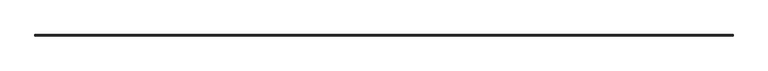
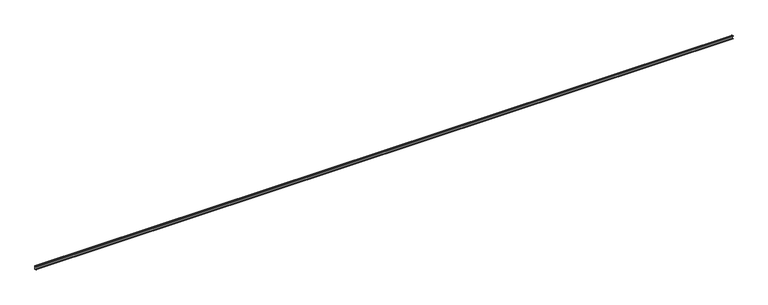
"""IFC4 building model written with IfcOpenShell, lengths in millimetres: beam geometry, 0912_Steel Framing_LC_KDS3530 : H_SB_AR_B03_LC-200x75x25x3.2."""

from ifc_helpers import new_model, si_unit, point, frame, frame_2d, origin, place, context, project, spatial, polyline, circle_curve, trimmed, segment, composite_curve, outline, extrude, source, transform, mapped, element, save


def beam_ae6eba6b(model_context):
    return source(origin(), model_context, "Body", "SweptSolid", [
        extrude(outline(composite_curve([segment(polyline([(18.6, 87.5), (18.6, -87.5)]), True, "CONTINUOUS"), segment(trimmed(circle_curve(frame_2d((6.1, -87.5)), 12.5), [point((18.6, -87.5))], [point((6.1, -100.0))], False, "CARTESIAN"), True, "CONTINUOUS"), segment(polyline([(6.1, -100.0), (-43.9, -100.0)]), True, "CONTINUOUS"), segment(trimmed(circle_curve(frame_2d((-43.9, -87.5)), 12.5), [point((-43.9, -100.0))], [point((-56.4, -87.5))], False, "CARTESIAN"), True, "CONTINUOUS"), segment(polyline([(-56.4, -87.5), (-56.4, -75.0), (-51.9, -75.0), (-51.9, -87.5)]), True, "CONTINUOUS"), segment(trimmed(circle_curve(frame_2d((-43.9, -87.5)), 8.0), [point((-51.9, -87.5))], [point((-43.9, -95.5))], True, "CARTESIAN"), True, "CONTINUOUS"), segment(polyline([(-43.9, -95.5), (6.1, -95.5)]), True, "CONTINUOUS"), segment(trimmed(circle_curve(frame_2d((6.1, -87.5)), 8.0), [point((6.1, -95.5))], [point((14.1, -87.5))], True, "CARTESIAN"), True, "CONTINUOUS"), segment(polyline([(14.1, -87.5), (14.1, 87.5)]), True, "CONTINUOUS"), segment(trimmed(circle_curve(frame_2d((6.1, 87.5)), 8.0), [point((14.1, 87.5))], [point((6.1, 95.5))], True, "CARTESIAN"), True, "CONTINUOUS"), segment(polyline([(6.1, 95.5), (-41.1, 95.5)]), True, "CONTINUOUS"), segment(trimmed(circle_curve(frame_2d((-41.1, 87.5)), 8.0), [point((-41.1, 95.5))], [point((-49.1, 87.5))], True, "CARTESIAN"), True, "CONTINUOUS"), segment(polyline([(-49.1, 87.5), (-49.1, 75.0), (-53.6, 75.0), (-53.6, 87.5)]), True, "CONTINUOUS"), segment(trimmed(circle_curve(frame_2d((-41.1, 87.5)), 12.5), [point((-53.6, 87.5))], [point((-41.1, 100.0))], False, "CARTESIAN"), True, "CONTINUOUS"), segment(polyline([(-41.1, 100.0), (6.1, 100.0)]), True, "CONTINUOUS"), segment(trimmed(circle_curve(frame_2d((6.1, 87.5)), 12.5), [point((6.1, 100.0))], [point((18.6, 87.5))], False, "CARTESIAN"), True, "CONTINUOUS")], self_intersect=False)), frame((-19950.0, 0.0, 0.0), z_axis=(1.0, 0.0, 0.0), x_axis=(0.0, 1.0, 0.0)), (0.0, 0.0, 1.0), 39450.0),
    ])


if __name__ == "__main__":
    model = new_model("IFC4")
    model_context = context("Model", 3, world=origin())
    ifc_project = project(units=[si_unit("LENGTHUNIT", "METRE", prefix="MILLI")], contexts=[model_context])
    site = spatial("IfcSite", under=ifc_project)
    building = spatial("IfcBuilding", under=site)
    placement = place(None, origin())
    beam_shape = beam_ae6eba6b(model_context)
    element("IfcBeam", 1, ObjectType="0912_Steel Framing_LC_KDS3530 : H_SB_AR_B03_LC-200x75x25x3.2", at=placement, inside=building, context=model_context, shape_type="MappedRepresentation", body=[
        mapped(beam_shape, transform((0.0, 0.0, 0.0), x_axis=(1.0, 0.0, 0.0), y_axis=(0.0, 1.0, 0.0), z_axis=(0.0, 0.0, 1.0))),
    ])
    save(model, "model.ifc")

# Revit data of these elements
# Type "0912_Steel Framing_LC_KDS3530 : H_SB_AR_B03_LC-200x75x25x3.2"
#   r = 8 mm
#   d = 25 mm
#   R = 11.2 mm
#   Perimeter = 0.78 m²/m
#   Nominal Weight = 14.00 kgf/m
#   Length [instance default] = 1000 mm
#   B = 75 mm
#   H = 200 mm
#   tw = 3.2 mm
#   x = 18.6 mm
#   A = 1.00 m²
#   Structural Material [instance default] = Steel, 45-345
#   Assembly Code = ""
# Element 1 (IfcBeam, "0912_Steel Framing_LC_KDS3530 : H_SB_AR_B03_LC-200x75x25x3.2")
#   Materials on its faces: "Steel, 45-345"
# Materials
#   "Steel, 45-345": class "Metal", colour RGB 189 187 185, transparency 0, Description = "Steel 345 MPa", Cost = 0
